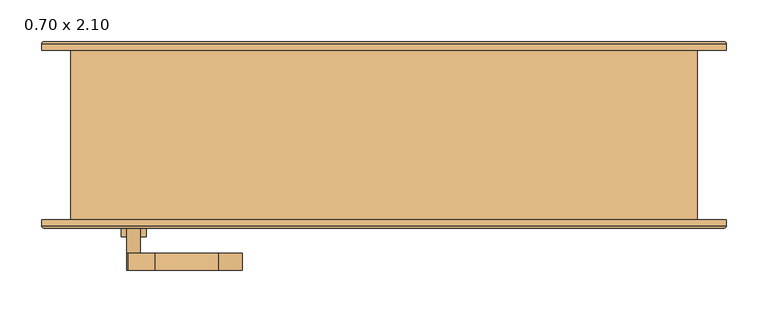
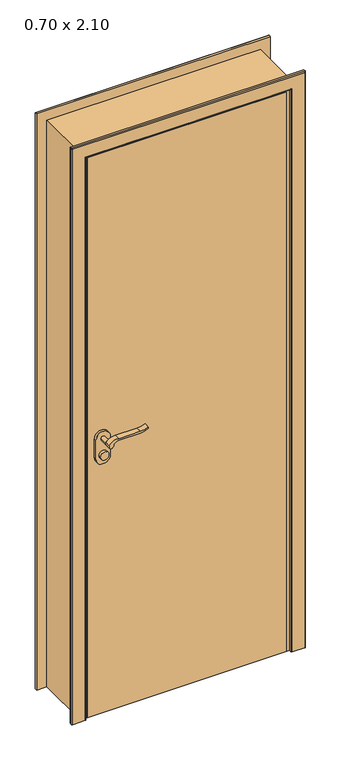
"""IFC4 building model written with IfcOpenShell, lengths in millimetres: door geometry, .CC_ND 300_PORTA SIMPLES DE ABRIR_COM EXTENSÃO : 0.70 x 2.10."""

from ifc_helpers import new_model, si_unit, point, frame, frame_2d, origin, origin_with_axes, place, context, project, spatial, polyline, circle_curve, ellipse_curve, trimmed, segment, composite_curve, outline, extrude, faceted_brep, source, transform, mapped, element, save
from ifc_brep_helpers import plane_surface, cylinder_surface, advanced_brep


def door_0_70_x_2_10_0ff34c02(model_context):
    return source(origin(), model_context, "Body", "SolidModel", [
        extrude(outline(composite_curve([segment(trimmed(circle_curve(frame_2d((964.5, -300.0)), 15.0), [point((964.5, -285.0))], [point((964.5, -315.0))], False, "CARTESIAN"), True, "CONTINUOUS"), segment(trimmed(circle_curve(frame_2d((964.5, -300.0)), 15.0), [point((964.5, -315.0))], [point((964.5, -285.0))], False, "CARTESIAN"), True, "CONTINUOUS")], self_intersect=False)), frame((0.0, -136.4, 0.0), z_axis=(0.0, 1.0, 0.0), x_axis=(0.0, 0.0, 1.0)), (0.0, 0.0, 1.0), 10.0),
        extrude(outline(composite_curve([segment(trimmed(circle_curve(frame_2d((964.5, -300.0)), 15.0), [point((964.5, -285.0))], [point((964.5, -315.0))], False, "CARTESIAN"), True, "CONTINUOUS"), segment(trimmed(circle_curve(frame_2d((964.5, -300.0)), 15.0), [point((964.5, -315.0))], [point((964.5, -285.0))], False, "CARTESIAN"), True, "CONTINUOUS")], self_intersect=False)), frame((0.0, -76.4, 0.0), z_axis=(0.0, 1.0, 0.0), x_axis=(0.0, 0.0, 1.0)), (0.0, 0.0, 1.0), 10.0),
        extrude(outline(composite_curve([segment(trimmed(circle_curve(frame_2d((1024.5, -300.0)), 8.0), [point((1029.1523287, -306.5081363))], [point((1024.5, -292.0))], False, "CARTESIAN"), True, "CONTINUOUS"), segment(trimmed(circle_curve(frame_2d((1019.3738613, -274.6138099)), 18.1261387), [point((1024.5, -292.0))], [point((1037.5, -274.6138099))], True, "CARTESIAN"), True, "CONTINUOUS"), segment(polyline([(1037.5, -274.6138099), (1037.5, -198.3564091)]), True, "CONTINUOUS"), segment(trimmed(circle_curve(frame_2d((1096.7709207, -201.9396612)), 59.3791355), [point((1037.5, -198.3564091))], [point((1046.7135558, -170.0))], False, "CARTESIAN"), True, "CONTINUOUS"), segment(polyline([(1046.7135558, -170.0), (1049.5, -170.0)]), True, "CONTINUOUS"), segment(trimmed(circle_curve(frame_2d((1127.7850638, -198.4227909)), 83.2850902), [point((1049.5, -170.0))], [point((1044.5, -198.3564091))], True, "CARTESIAN"), True, "CONTINUOUS"), segment(polyline([(1044.5, -198.3564091), (1044.5, -274.6325667)]), True, "CONTINUOUS"), segment(trimmed(circle_curve(frame_2d((1007.2555521, -276.3324871)), 37.2832219), [point((1044.5, -274.6325667))], [point((1029.1523287, -306.5081363))], False, "CARTESIAN"), True, "CONTINUOUS")], self_intersect=False)), frame((0.0, -176.4, 0.0), z_axis=(0.0, 1.0, 0.0), x_axis=(0.0, 0.0, 1.0)), (0.0, 0.0, 1.0), 20.0),
        extrude(outline(composite_curve([segment(trimmed(circle_curve(frame_2d((1019.3738682, -274.6138122)), 18.1261318), [point((1024.4999903, -292.0))], [point((1037.5, -274.6138122))], True, "CARTESIAN"), True, "CONTINUOUS"), segment(polyline([(1037.5, -274.6138122), (1037.5, -198.3564091)]), True, "CONTINUOUS"), segment(trimmed(circle_curve(frame_2d((1096.7709207, -201.9396612)), 59.3791355), [point((1037.5, -198.3564091))], [point((1046.7135558, -170.0))], False, "CARTESIAN"), True, "CONTINUOUS"), segment(polyline([(1046.7135558, -170.0), (1049.5, -170.0)]), True, "CONTINUOUS"), segment(trimmed(circle_curve(frame_2d((1127.7850638, -198.4227909)), 83.2850902), [point((1049.5, -170.0))], [point((1044.5, -198.3564091))], True, "CARTESIAN"), True, "CONTINUOUS"), segment(polyline([(1044.5, -198.3564091), (1044.5, -274.6325667)]), True, "CONTINUOUS"), segment(trimmed(circle_curve(frame_2d((1007.2555521, -276.3324871)), 37.2832219), [point((1044.5, -274.6325667))], [point((1029.1523287, -306.5081363))], False, "CARTESIAN"), True, "CONTINUOUS"), segment(trimmed(circle_curve(frame_2d((1024.5, -300.0)), 8.0), [point((1029.1523287, -306.5081363))], [point((1024.4999903, -292.0))], False, "CARTESIAN"), True, "CONTINUOUS")], self_intersect=False)), frame((0.0, -46.4, 0.0), z_axis=(0.0, 1.0, 0.0), x_axis=(0.0, 0.0, 1.0)), (0.0, 0.0, 1.0), 20.0),
        extrude(outline(composite_curve([segment(trimmed(circle_curve(frame_2d((1024.5, -300.0)), 8.0), [point((1024.5, -292.0))], [point((1024.5, -308.0))], False, "CARTESIAN"), True, "CONTINUOUS"), segment(trimmed(circle_curve(frame_2d((1024.5, -300.0)), 8.0), [point((1024.5, -308.0))], [point((1024.5, -292.0))], False, "CARTESIAN"), True, "CONTINUOUS")], self_intersect=False)), frame((0.0, -156.4, 0.0), z_axis=(0.0, 1.0, 0.0), x_axis=(0.0, 0.0, 1.0)), (0.0, 0.0, 1.0), 30.0),
        extrude(outline(composite_curve([segment(trimmed(circle_curve(frame_2d((1024.5, -300.0)), 8.0), [point((1024.5, -292.0))], [point((1024.5, -308.0))], False, "CARTESIAN"), True, "CONTINUOUS"), segment(trimmed(circle_curve(frame_2d((1024.5, -300.0)), 8.0), [point((1024.5, -308.0))], [point((1024.5, -292.0))], False, "CARTESIAN"), True, "CONTINUOUS")], self_intersect=False)), frame((0.0, -76.4, 0.0), z_axis=(0.0, 1.0, 0.0), x_axis=(0.0, 0.0, 1.0)), (0.0, 0.0, 1.0), 30.0),
        extrude(outline(composite_curve([segment(trimmed(circle_curve(frame_2d((954.5, -300.0)), 25.0), [point((954.5, -325.0))], [point((954.5, -275.0))], False, "CARTESIAN"), True, "CONTINUOUS"), segment(polyline([(954.5, -275.0), (1024.5, -275.0)]), True, "CONTINUOUS"), segment(trimmed(circle_curve(frame_2d((1024.5, -300.0)), 25.0), [point((1024.5, -275.0))], [point((1024.5, -325.0))], False, "CARTESIAN"), True, "CONTINUOUS"), segment(polyline([(1024.5, -325.0), (954.5, -325.0)]), True, "CONTINUOUS")], self_intersect=False)), frame((0.0, -126.4, 0.0), z_axis=(0.0, 1.0, 0.0), x_axis=(0.0, 0.0, 1.0)), (0.0, 0.0, 1.0), 10.0),
        extrude(outline(composite_curve([segment(trimmed(circle_curve(frame_2d((954.5, -300.0)), 25.0), [point((954.5, -325.0))], [point((954.5, -275.0))], False, "CARTESIAN"), True, "CONTINUOUS"), segment(polyline([(954.5, -275.0), (1024.5, -275.0)]), True, "CONTINUOUS"), segment(trimmed(circle_curve(frame_2d((1024.5, -300.0)), 25.0), [point((1024.5, -275.0))], [point((1024.5, -325.0))], False, "CARTESIAN"), True, "CONTINUOUS"), segment(polyline([(1024.5, -325.0), (954.5, -325.0)]), True, "CONTINUOUS")], self_intersect=False)), frame((0.0, -86.4, 0.0), z_axis=(0.0, 1.0, 0.0), x_axis=(0.0, 0.0, 1.0)), (0.0, 0.0, 1.0), 10.0),
        advanced_brep(
        [(-410.0, -116.4, 0.0), (-360.0, -116.4, 0.0), (-360.0, -123.4, 0.0), (-363.0, -126.4, 0.0), (-407.0, -126.4, 0.0), (-410.0, -123.4, 0.0), (-410.0, -116.4, 2135.0), (410.0, -116.4, 2135.0), (410.0, -116.4, 0.0), (360.0, -116.4, 0.0), (360.0, -116.4, 2085.0), (-360.0, -116.4, 2085.0), (-360.0, -123.4, 2085.0), (-363.0, -126.4, 2088.0), (363.0, -126.4, 2088.0), (363.0, -126.4, 0.0), (407.0, -126.4, 0.0), (407.0, -126.4, 2132.0), (-407.0, -126.4, 2132.0), (-410.0, -123.4, 2135.0), (410.0, -123.4, 2135.0), (410.0, -123.4, 0.0), (360.0, -123.4, 0.0), (360.0, -123.4, 2085.0)],
        [
            (0, 1),
            (1, 2),
            (2, 3, circle_curve(frame((-363.0, -123.4, 0.0), z_axis=(0.0, 0.0, -1.0), x_axis=(1.0, 0.0, 0.0)), 3.0)),
            (3, 4),
            (4, 5, circle_curve(frame((-407.0, -123.4, 0.0), z_axis=(0.0, 0.0, -1.0), x_axis=(1.0, 0.0, 0.0)), 3.0)),
            (5, 0),
            (0, 6),
            (6, 7),
            (7, 8),
            (8, 9),
            (9, 10),
            (10, 11),
            (11, 1),
            (11, 12),
            (12, 2),
            (12, 13, ellipse_curve(frame((-363.0, -123.4, 2088.0), z_axis=(-0.7071067811865475, 0.0, -0.7071067811865475), x_axis=(0.7071067811865474, 0.0, -0.7071067811865476)), 4.2426407, 3.0)),
            (13, 3),
            (13, 14),
            (14, 15),
            (15, 16),
            (16, 17),
            (17, 18),
            (18, 4),
            (18, 19, ellipse_curve(frame((-407.0, -123.4, 2132.0), z_axis=(-0.7071067811865475, 0.0, -0.7071067811865475), x_axis=(0.7071067811865474, 0.0, -0.7071067811865476)), 4.2426407, 3.0)),
            (19, 5),
            (19, 6),
            (7, 20),
            (20, 21),
            (21, 8),
            (21, 16, circle_curve(frame((407.0, -123.4, 0.0), z_axis=(0.0, 0.0, -1.0), x_axis=(-1.0, 0.0, 0.0)), 3.0)),
            (15, 22, circle_curve(frame((363.0, -123.4, 0.0), z_axis=(0.0, 0.0, -1.0), x_axis=(-1.0, 0.0, 0.0)), 3.0)),
            (22, 9),
            (23, 10),
            (22, 23),
            (14, 23, ellipse_curve(frame((363.0, -123.4, 2088.0), z_axis=(0.7071067811865475, 0.0, -0.7071067811865475), x_axis=(0.7071067811865474, 0.0, 0.7071067811865476)), 4.2426407, 3.0)),
            (20, 17, ellipse_curve(frame((407.0, -123.4, 2132.0), z_axis=(0.7071067811865475, 0.0, -0.7071067811865475), x_axis=(0.7071067811865474, 0.0, 0.7071067811865476)), 4.2426407, 3.0)),
            (23, 12),
            (19, 20),
        ],
        [
            plane_surface(frame((-360.0, -116.4, 0.0), z_axis=(0.0, 0.0, -1.0), x_axis=(0.0, 1.0, 0.0))),
            plane_surface(frame((-410.0, -116.4, 0.0), z_axis=(0.0, 1.0, 0.0), x_axis=(0.0, 0.0, 1.0))),
            plane_surface(frame((-360.0, -116.4, 0.0), z_axis=(1.0, 0.0, 0.0), x_axis=(0.0, 0.0, 1.0))),
            cylinder_surface(frame((-363.0, -123.4, 0.0), z_axis=(0.0, 0.0, -1.0), x_axis=(1.0, 0.0, 0.0)), 3.0),
            plane_surface(frame((-363.0, -126.4, 0.0), z_axis=(0.0, -1.0, 0.0), x_axis=(0.0, 0.0, 1.0))),
            cylinder_surface(frame((-407.0, -123.4, 0.0), z_axis=(0.0, 0.0, -1.0), x_axis=(1.0, 0.0, 0.0)), 3.0),
            plane_surface(frame((-410.0, -123.4, 0.0), z_axis=(-1.0, 0.0, 0.0), x_axis=(0.0, 0.0, 1.0))),
            plane_surface(frame((410.0, -123.4, 2135.0), z_axis=(1.0, 0.0, 0.0), x_axis=(0.0, 0.0, -1.0))),
            plane_surface(frame((360.0, -116.4, 0.0), z_axis=(0.0, 0.0, -1.0), x_axis=(0.0, 1.0, 0.0))),
            plane_surface(frame((360.0, -116.4, 2085.0), z_axis=(-1.0, 0.0, 0.0), x_axis=(0.0, 0.0, -1.0))),
            cylinder_surface(frame((363.0, -123.4, 2085.0), z_axis=(0.0, 0.0, 1.0), x_axis=(-1.0, 0.0, 0.0)), 3.0),
            cylinder_surface(frame((407.0, -123.4, 2085.0), z_axis=(0.0, 0.0, 1.0), x_axis=(-1.0, 0.0, 0.0)), 3.0),
            plane_surface(frame((-360.0, -116.4, 2085.0), z_axis=(0.0, 0.0, -1.0), x_axis=(1.0, 0.0, 0.0))),
            plane_surface(frame((-410.0, -123.4, 2135.0), z_axis=(0.0, 0.0, 1.0), x_axis=(1.0, 0.0, 0.0))),
            cylinder_surface(frame((-360.0, -123.4, 2088.0), z_axis=(-1.0, 0.0, 0.0), x_axis=(0.0, 0.0, -1.0)), 3.0),
            cylinder_surface(frame((-360.0, -123.4, 2132.0), z_axis=(-1.0, 0.0, 0.0), x_axis=(0.0, 0.0, -1.0)), 3.0),
        ],
        [
            (0, [[1, 2, 3, 4, 5, 6]]),
            (1, [[-1, 7, 8, 9, 10, 11, 12, 13]]),
            (2, [[-2, -13, 14, 15]]),
            (3, [[-3, -15, 16, 17]]),
            (4, [[-4, -17, 18, 19, 20, 21, 22, 23]]),
            (5, [[-5, -23, 24, 25]]),
            (6, [[-6, -25, 26, -7]]),
            (7, [[27, 28, 29, -9]]),
            (8, [[-29, 30, -20, 31, 32, -10]]),
            (9, [[33, -11, -32, 34]]),
            (10, [[35, -34, -31, -19]]),
            (11, [[36, -21, -30, -28]]),
            (12, [[-14, -12, -33, 37]]),
            (13, [[-26, 38, -27, -8]]),
            (14, [[-16, -37, -35, -18]]),
            (15, [[-24, -22, -36, -38]]),
        ],
    ),
        advanced_brep(
        [(410.0, 86.9, 0.0), (360.0, 86.9, 0.0), (360.0, 93.9157283, 0.0), (362.9842717, 96.9, 0.0), (407.0342217, 96.9, 0.0), (410.0, 93.9342217, 0.0), (410.0, 86.9, 2135.0), (-410.0, 86.9, 2135.0), (-410.0, 86.9, 0.0), (-360.0, 86.9, 0.0), (-360.0, 86.9, 2085.0), (360.0, 86.9, 2085.0), (360.0, 93.9157283, 2085.0), (362.9842717, 96.9, 2087.9842717), (-362.9842717, 96.9, 2087.9842717), (-362.9842717, 96.9, 0.0), (-407.0342217, 96.9, 0.0), (-407.0342217, 96.9, 2132.0342217), (407.0342217, 96.9, 2132.0342217), (410.0, 93.9342217, 2135.0), (-410.0, 93.9342217, 2135.0), (-410.0, 93.9342217, 0.0), (-360.0, 93.9157283, 0.0), (-360.0, 93.9157283, 2085.0)],
        [
            (0, 1),
            (1, 2),
            (2, 3, circle_curve(frame((362.9842717, 93.9157283, 0.0), z_axis=(0.0, 0.0, -1.0), x_axis=(1.0, 0.0, 0.0)), 2.9842717)),
            (3, 4),
            (4, 5, circle_curve(frame((407.0342217, 93.9342217, 0.0), z_axis=(0.0, 0.0, -1.0), x_axis=(1.0, 0.0, 0.0)), 2.9657783)),
            (5, 0),
            (0, 6),
            (6, 7),
            (7, 8),
            (8, 9),
            (9, 10),
            (10, 11),
            (11, 1),
            (11, 12),
            (12, 2),
            (12, 13, ellipse_curve(frame((362.9842717, 93.9157283, 2087.9842717), z_axis=(0.7071067811865475, 0.0, -0.7071067811865475), x_axis=(-0.7071067811865474, 0.0, -0.7071067811865476)), 4.2203975, 2.9842717)),
            (13, 3),
            (13, 14),
            (14, 15),
            (15, 16),
            (16, 17),
            (17, 18),
            (18, 4),
            (18, 19, ellipse_curve(frame((407.0342217, 93.9342217, 2132.0342217), z_axis=(0.7071067811865475, 0.0, -0.7071067811865475), x_axis=(-0.7071067811865474, 0.0, -0.7071067811865476)), 4.1942438, 2.9657783)),
            (19, 5),
            (19, 6),
            (7, 20),
            (20, 21),
            (21, 8),
            (21, 16, circle_curve(frame((-407.0342217, 93.9342217, 0.0), z_axis=(0.0, 0.0, -1.0), x_axis=(-1.0, 0.0, 0.0)), 2.9657783)),
            (15, 22, circle_curve(frame((-362.9842717, 93.9157283, 0.0), z_axis=(0.0, 0.0, -1.0), x_axis=(-1.0, 0.0, 0.0)), 2.9842717)),
            (22, 9),
            (23, 10),
            (22, 23),
            (14, 23, ellipse_curve(frame((-362.9842717, 93.9157283, 2087.9842717), z_axis=(-0.7071067811865475, 0.0, -0.7071067811865475), x_axis=(-0.7071067811865474, 0.0, 0.7071067811865476)), 4.2203975, 2.9842717)),
            (20, 17, ellipse_curve(frame((-407.0342217, 93.9342217, 2132.0342217), z_axis=(-0.7071067811865475, 0.0, -0.7071067811865475), x_axis=(-0.7071067811865474, 0.0, 0.7071067811865476)), 4.1942438, 2.9657783)),
            (23, 12),
            (19, 20),
        ],
        [
            plane_surface(frame((360.0, 86.9, 0.0), z_axis=(0.0, 0.0, -1.0), x_axis=(0.0, 1.0, 0.0))),
            plane_surface(frame((410.0, 86.9, 0.0), z_axis=(0.0, -1.0, 0.0), x_axis=(0.0, 0.0, 1.0))),
            plane_surface(frame((360.0, 86.9, 0.0), z_axis=(-1.0, 0.0, 0.0), x_axis=(0.0, 0.0, 1.0))),
            cylinder_surface(frame((362.9842717, 93.9157283, 0.0), z_axis=(0.0, 0.0, -1.0), x_axis=(1.0, 0.0, 0.0)), 2.9842717),
            plane_surface(frame((362.9842717, 96.9, 0.0), z_axis=(0.0, 1.0, 0.0), x_axis=(0.0, 0.0, 1.0))),
            cylinder_surface(frame((407.0342217, 93.9342217, 0.0), z_axis=(0.0, 0.0, -1.0), x_axis=(1.0, 0.0, 0.0)), 2.9657783),
            plane_surface(frame((410.0, 93.9342217, 0.0), z_axis=(1.0, 0.0, 0.0), x_axis=(0.0, 0.0, 1.0))),
            plane_surface(frame((-410.0, 93.9342217, 2135.0), z_axis=(-1.0, 0.0, 0.0), x_axis=(0.0, 0.0, -1.0))),
            plane_surface(frame((-360.0, 86.9, 0.0), z_axis=(0.0, 0.0, -1.0), x_axis=(0.0, 1.0, 0.0))),
            plane_surface(frame((-360.0, 86.9, 2085.0), z_axis=(1.0, 0.0, 0.0), x_axis=(0.0, 0.0, -1.0))),
            cylinder_surface(frame((-362.9842717, 93.9157283, 2085.0), z_axis=(0.0, 0.0, 1.0), x_axis=(-1.0, 0.0, 0.0)), 2.9842717),
            cylinder_surface(frame((-407.0342217, 93.9342217, 2085.0), z_axis=(0.0, 0.0, 1.0), x_axis=(-1.0, 0.0, 0.0)), 2.9657783),
            plane_surface(frame((360.0, 86.9, 2085.0), z_axis=(0.0, 0.0, -1.0), x_axis=(-1.0, 0.0, 0.0))),
            plane_surface(frame((410.0, 93.9342217, 2135.0), z_axis=(0.0, 0.0, 1.0), x_axis=(-1.0, 0.0, 0.0))),
            cylinder_surface(frame((360.0, 93.9157283, 2087.9842717), z_axis=(1.0, 0.0, 0.0), x_axis=(0.0, 0.0, 1.0)), 2.9842717),
            cylinder_surface(frame((360.0, 93.9342217, 2132.0342217), z_axis=(1.0, 0.0, 0.0), x_axis=(0.0, 0.0, 1.0)), 2.9657783),
        ],
        [
            (0, [[1, 2, 3, 4, 5, 6]]),
            (1, [[-1, 7, 8, 9, 10, 11, 12, 13]]),
            (2, [[-2, -13, 14, 15]]),
            (3, [[-3, -15, 16, 17]]),
            (4, [[-4, -17, 18, 19, 20, 21, 22, 23]]),
            (5, [[-5, -23, 24, 25]]),
            (6, [[-6, -25, 26, -7]]),
            (7, [[27, 28, 29, -9]]),
            (8, [[-29, 30, -20, 31, 32, -10]]),
            (9, [[33, -11, -32, 34]]),
            (10, [[35, -34, -31, -19]]),
            (11, [[36, -21, -30, -28]]),
            (12, [[-14, -12, -33, 37]]),
            (13, [[-26, 38, -27, -8]]),
            (14, [[-16, -37, -35, -18]]),
            (15, [[-24, -22, -36, -38]]),
        ],
    ),
        faceted_brep([(342.0, 86.9, 0.0), (375.0, 86.9, 0.0), (375.0, -116.4, 0.0), (350.0, -116.4, 0.0), (350.0, -86.4, 0.0), (342.0, -86.4, 0.0), (342.0, 86.9, 2067.0), (-342.0, 86.9, 2067.0), (-342.0, 86.9, 0.0), (-375.0, 86.9, 0.0), (-375.0, 86.9, 2100.0), (375.0, 86.9, 2100.0), (375.0, -116.4, 2100.0), (-375.0, -116.4, 2100.0), (-375.0, -116.4, 0.0), (-350.0, -116.4, 0.0), (-350.0, -116.4, 2075.0), (350.0, -116.4, 2075.0), (350.0, -86.4, 2075.0), (-350.0, -86.4, 2075.0), (-350.0, -86.4, 0.0), (-342.0, -86.4, 0.0), (-342.0, -86.4, 2067.0), (342.0, -86.4, 2067.0)], [[[0, 1, 2, 3, 4, 5]], [[1, 0, 6, 7, 8, 9, 10, 11]], [[2, 1, 11, 12]], [[3, 2, 12, 13, 14, 15, 16, 17]], [[4, 3, 17, 18]], [[5, 4, 18, 19, 20, 21, 22, 23]], [[0, 5, 23, 6]], [[7, 22, 21, 8]], [[8, 21, 20, 15, 14, 9]], [[13, 10, 9, 14]], [[19, 16, 15, 20]], [[12, 11, 10, 13]], [[18, 17, 16, 19]], [[6, 23, 22, 7]]]),
        extrude(outline(polyline([(-350.0, -86.4), (350.0, -86.4), (350.0, -116.4), (-350.0, -116.4), (-350.0, -86.4)])), origin_with_axes(), (0.0, 0.0, 1.0), 2075.0),
    ])


if __name__ == "__main__":
    model = new_model("IFC4")
    model_context = context("Model", 3, world=origin())
    ifc_project = project(units=[si_unit("LENGTHUNIT", "METRE", prefix="MILLI")], contexts=[model_context])
    site = spatial("IfcSite", under=ifc_project)
    building = spatial("IfcBuilding", under=site)
    placement = place(None, origin())
    door_0_70_x_2_10_shape = door_0_70_x_2_10_0ff34c02(model_context)
    element("IfcDoor", 1, ObjectType=".CC_ND 300_PORTA SIMPLES DE ABRIR_COM EXTENSÃO : 0.70 x 2.10", at=placement, inside=building, context=model_context, shape_type="MappedRepresentation", body=[
        mapped(door_0_70_x_2_10_shape, transform((0.0, 0.0, 0.0), x_axis=(1.0, 0.0, 0.0), y_axis=(0.0, 1.0, 0.0), z_axis=(0.0, 0.0, 1.0))),
    ])
    save(model, "model.ifc")

# Revit data of these elements
# Type ".CC_ND 300_PORTA SIMPLES DE ABRIR_COM EXTENSÃO : 0.70 x 2.10"
#   Type Mark = "155"
#   Rough Width = 0.75 m
#   Espessura moldura externa = 0.01 m
#   Espessura moldura interna = 0.01 m
#   Largura moldura = 0.05 m
#   Extensão acabamento exterior [instance default] = 0.00 m
#   Extensão acabamento interior [instance default] = 0.00 m
#   Espessura batente = 0.025 m
#   Thickness = 0.03 m
#   Altura batente = 2.085 m
#   Aux Arco [instance default] = 0.70 m
#   Rough Height = 2.125 m
#   Height = 2.10 m
#   Width = 0.70 m
#   Moldura interna [instance default] = yes
#   Moldura externa [instance default] = yes
#   Porta = .MADEIRA COM PINTURA ESMALTE BRANCO ACETINADO
#   Moldura = .MADEIRA COM PINTURA ESMALTE BRANCO ACETINADO
#   Maçaneta = .ALUMÍNIO
#   Batente = .MADEIRA COM PINTURA ESMALTE BRANCO ACETINADO
#   Function = (empty or 0)
#   Wall Closure = (empty or 0)
# Element 1 (IfcDoor, ".CC_ND 300_PORTA SIMPLES DE ABRIR_COM EXTENSÃO : 0.70 x 2.10")
#   Extensão acabamento interior = 0.0295 m
#   Aux Arco = 0.7295 m
#   Materials on its faces: ".MADEIRA COM PINTURA ESMALTE BRANCO ACETINADO", ".ALUMÍNIO"
# Materials
#   ".MADEIRA COM PINTURA ESMALTE BRANCO ACETINADO": class ".CC_MADEIRAS", colour RGB 240 240 240, transparency 0, Description = "Madeira com pintura esmalte branco acetinado.", Cost = 0
#   ".ALUMÍNIO": class "CC_METAIS", colour RGB 244 244 244, transparency 0, Description = "Material alumínio", Cost = 0
